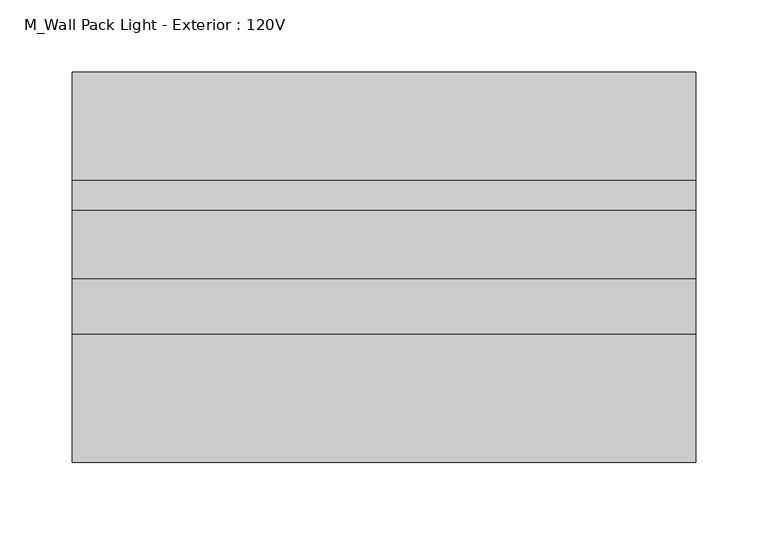
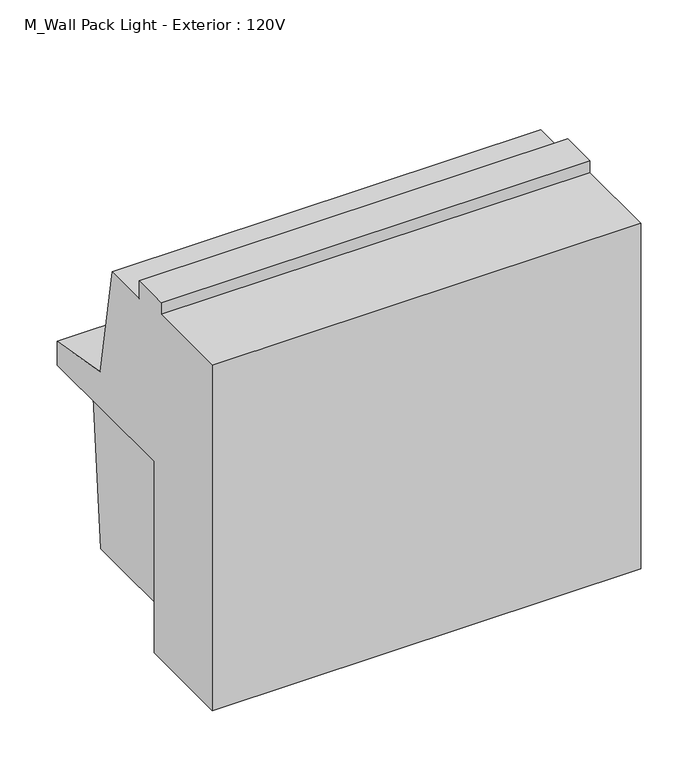
"""IFC4 building model written with IfcOpenShell, lengths in millimetres: light fixture geometry, M_Wall Pack Light - Exterior : 120V."""

import ifcopenshell
import ifcopenshell.guid

model = None  # the IFC model being written
_history = None  # IfcOwnerHistory: only IFC2X3 demands one
_inside = {}  # id of a spatial element -> (the spatial element, [elements in it])
_under = {}  # id of a project, library or spatial element -> (it, [spatial elements below it])
_declared = {}  # id of a project -> (the project, [libraries it declares])
_typed = {}  # id of a type object -> (the type object, [elements of that type])
_made_of = {}  # id of a material, layer set ... -> (it, [elements and type objects made of it])


def new_model(schema):
    """Start an empty IFC model of exactly this schema.

    Asked for "IFC4X3", IfcOpenShell would pick the latest addendum, in which some entities
    have other attributes; the version numbers below select the first issue.
    IFC2X3 requires an IfcOwnerHistory on every rooted entity: one is made here for all.
    """
    global model, _history
    if schema == "IFC4X3":
        model = ifcopenshell.file(schema_version=(4, 3, 0, 0))
    else:
        model = ifcopenshell.file(schema=schema)
    _inside.clear()
    _under.clear()
    _declared.clear()
    _typed.clear()
    _made_of.clear()
    _history = None
    if model.schema == "IFC2X3":
        org = make("IfcOrganization", Name="unknown")
        user = make(
            "IfcPersonAndOrganization",
            ThePerson=make("IfcPerson", FamilyName="unknown"),
            TheOrganization=org,
        )
        app = make(
            "IfcApplication",
            ApplicationDeveloper=org,
            Version="unknown",
            ApplicationFullName="unknown",
            ApplicationIdentifier="unknown",
        )
        _history = make(
            "IfcOwnerHistory",
            OwningUser=user,
            OwningApplication=app,
            ChangeAction="ADDED",
            CreationDate=0,
        )
    return model


def make(cls, **values):
    """One entity of the class cls with the attributes given. An attribute that is None is left unset."""
    return model.create_entity(
        cls, **{name: value for name, value in values.items() if value is not None}
    )


def rooted(cls, **values):
    """An entity with a GlobalId (a new one), such as an element, a storey or a relation."""
    return make(cls, GlobalId=ifcopenshell.guid.new(), OwnerHistory=_history, **values)


def si_unit(unit_type, name, prefix=None):
    """IfcSIUnit, for example si_unit("LENGTHUNIT", "METRE", prefix="MILLI")."""
    return make("IfcSIUnit", UnitType=unit_type, Prefix=prefix, Name=name)


def assignment(units):
    """IfcUnitAssignment: the units of a project."""
    return None if units is None else make("IfcUnitAssignment", Units=units)


def point(xyz):
    """IfcCartesianPoint."""
    return None if xyz is None else make("IfcCartesianPoint", Coordinates=xyz)


def direction(xyz):
    """IfcDirection."""
    return None if xyz is None else make("IfcDirection", DirectionRatios=xyz)


def frame(location, z_axis=None, x_axis=None):
    """IfcAxis2Placement3D, a coordinate frame: its origin and axes. An axis left out is left unset."""
    return make(
        "IfcAxis2Placement3D",
        Location=point(location),
        Axis=direction(z_axis),
        RefDirection=direction(x_axis),
    )


def origin():
    """The frame at (0, 0, 0) with its axes left unset."""
    return frame((0.0, 0.0, 0.0))


def place(relative_to, where):
    """IfcLocalPlacement: puts the frame where relative to a parent placement (None: the world)."""
    return make(
        "IfcLocalPlacement", PlacementRelTo=relative_to, RelativePlacement=where
    )


def context(
    kind, dimensions, precision=None, world=None, true_north=None, identifier=None
):
    """IfcGeometricRepresentationContext, for example the 3D "Model" context."""
    return make(
        "IfcGeometricRepresentationContext",
        ContextIdentifier=identifier,
        ContextType=kind,
        CoordinateSpaceDimension=dimensions,
        Precision=precision,
        WorldCoordinateSystem=world,
        TrueNorth=true_north,
    )


def project(units=None, contexts=None):
    """IfcProject with its units and contexts."""
    return rooted(
        "IfcProject",
        Name="project",
        RepresentationContexts=contexts,
        UnitsInContext=assignment(units),
    )


def spatial(cls, under=None, at=None, **own):
    """A site, building, storey or space (cls), placed at a placement, below another one or the project."""
    s = rooted(cls, ObjectPlacement=at, **own)
    if under is not None:
        _under.setdefault(under.id(), (under, []))[1].append(s)
    return s


def polyline(points):
    """IfcPolyline through the points."""
    return make("IfcPolyline", Points=[point(p) for p in points])


def outline(outer, holes=None, kind="AREA"):
    """IfcArbitraryClosedProfileDef: a profile drawn as a closed curve; with holes, ...WithVoids."""
    if holes is None:
        return make("IfcArbitraryClosedProfileDef", ProfileType=kind, OuterCurve=outer)
    return make(
        "IfcArbitraryProfileDefWithVoids",
        ProfileType=kind,
        OuterCurve=outer,
        InnerCurves=holes,
    )


def extrude(swept, where, along, depth):
    """IfcExtrudedAreaSolid: the profile swept, set in the frame where, extruded along a direction by depth."""
    return make(
        "IfcExtrudedAreaSolid",
        SweptArea=swept,
        Position=where,
        ExtrudedDirection=direction(along),
        Depth=depth,
    )


def shape(context_of_items, identifier, shape_type, items):
    """IfcShapeRepresentation: the items that make up one representation, for example the "Body"."""
    return make(
        "IfcShapeRepresentation",
        ContextOfItems=context_of_items,
        RepresentationIdentifier=identifier,
        RepresentationType=shape_type,
        Items=items,
    )


def source(mapping_origin, context_of_items, identifier, shape_type, items):
    """IfcRepresentationMap: a shape defined once, which mapped items show again and again."""
    return make(
        "IfcRepresentationMap",
        MappingOrigin=mapping_origin,
        MappedRepresentation=shape(context_of_items, identifier, shape_type, items),
    )


def transform(
    local_origin,
    x_axis=None,
    y_axis=None,
    z_axis=None,
    scale=None,
    scale2=None,
    scale3=None,
    uniform=True,
):
    """IfcCartesianTransformationOperator3D, or its non-uniform kind. x_axis, y_axis, z_axis: its Axis1, 2, 3."""
    if uniform:
        return make(
            "IfcCartesianTransformationOperator3D",
            Axis1=direction(x_axis),
            Axis2=direction(y_axis),
            LocalOrigin=point(local_origin),
            Scale=scale,
            Axis3=direction(z_axis),
        )
    return make(
        "IfcCartesianTransformationOperator3DnonUniform",
        Axis1=direction(x_axis),
        Axis2=direction(y_axis),
        LocalOrigin=point(local_origin),
        Scale=scale,
        Axis3=direction(z_axis),
        Scale2=scale2,
        Scale3=scale3,
    )


def mapped(mapping_source, mapping_target):
    """IfcMappedItem: shows the shape of a source again, moved by a transform."""
    return make(
        "IfcMappedItem", MappingSource=mapping_source, MappingTarget=mapping_target
    )


def made_of(thing, what):
    """Note that an element or type object is made of a material, layer set ...; save() writes the relation."""
    if what is not None:
        _made_of.setdefault(what.id(), (what, []))[1].append(thing)
    return thing


def element(
    cls,
    number,
    at=None,
    inside=None,
    cuts=None,
    type_object=None,
    material=None,
    context=None,
    identifier="Body",
    shape_type=None,
    held_by="IfcProductDefinitionShape",
    body=None,
    shapes=None,
    **own,
):
    """One element of the class cls, such as IfcWall. Its Tag is "e" and its number.

    at: its placement. inside: the storey or other place that contains it. cuts: it is an
    opening in that element (IfcRelVoidsElement). A single representation is given by context,
    identifier, shape_type and body (its items); several are given by shapes. held_by: the class
    of the entity that holds the representations. save() writes the other relations.
    """
    e = rooted(cls, Tag="e%d" % number, ObjectPlacement=at, **own)
    if body is not None:
        shapes = [shape(context, identifier, shape_type, body)]
    if shapes is not None:
        e.Representation = make(held_by, Representations=shapes)
    if inside is not None:
        _inside.setdefault(inside.id(), (inside, []))[1].append(e)
    if cuts is not None:
        rooted(
            "IfcRelVoidsElement", RelatingBuildingElement=cuts, RelatedOpeningElement=e
        )
    if type_object is not None:
        _typed.setdefault(type_object.id(), (type_object, []))[1].append(e)
    return made_of(e, material)


def aggregate(whole, parts):
    """IfcRelAggregates: a whole, such as a stair, and the parts it consists of."""
    return rooted("IfcRelAggregates", RelatingObject=whole, RelatedObjects=parts)


def save(model, path):
    """Write the relations noted so far, then the file.

    IfcRelAggregates (storeys below a building ...), IfcRelContainedInSpatialStructure (elements
    in a storey), IfcRelDefinesByType, IfcRelAssociatesMaterial and IfcRelDeclares: one each for
    every whole, place, type object, material and project.
    """
    for whole, parts in _under.values():
        aggregate(whole, parts)
    for where, things in _inside.values():
        rooted(
            "IfcRelContainedInSpatialStructure",
            RelatedElements=things,
            RelatingStructure=where,
        )
    for kind, things in _typed.values():
        rooted("IfcRelDefinesByType", RelatedObjects=things, RelatingType=kind)
    for what, things in _made_of.values():
        rooted("IfcRelAssociatesMaterial", RelatedObjects=things, RelatingMaterial=what)
    for by, libraries in _declared.values():
        rooted("IfcRelDeclares", RelatingContext=by, RelatedDefinitions=libraries)
    model.write(path)


def m_wall_pack_light_exterior_120v_7c12f8c9(model_context):
    return source(origin(), model_context, "Body", "SweptSolid", [
        extrude(outline(polyline([(365.820745, 2350.75), (228.6, 2350.75), (228.6, 2534.9), (380.9170754, 2534.9), (365.820745, 2350.75)])), frame((-68.7349223, 0.0, 0.0), z_axis=(1.0, 0.0, 0.0), x_axis=(0.0, 1.0, 0.0)), (0.0, 0.0, 1.0), 380.9989788),
        extrude(outline(polyline([(215.9, 2712.7), (254.0, 2712.7), (254.0, 2693.65), (301.440971, 2693.65), (322.4426549, 2574.5435323), (397.4850056, 2561.3115412), (397.4850056, 2535.9115412), (228.6, 2535.9115412), (228.6, 2331.7), (127.0, 2331.7), (127.0, 2700.0), (215.9, 2700.0), (215.9, 2712.7)])), frame((-94.1359435, 0.0, 0.0), z_axis=(1.0, 0.0, 0.0), x_axis=(0.0, 1.0, 0.0)), (0.0, 0.0, 1.0), 431.8),
    ])


if __name__ == "__main__":
    model = new_model("IFC4")
    model_context = context("Model", 3, world=origin())
    ifc_project = project(units=[si_unit("LENGTHUNIT", "METRE", prefix="MILLI")], contexts=[model_context])
    site = spatial("IfcSite", under=ifc_project)
    building = spatial("IfcBuilding", under=site)
    placement = place(None, origin())
    m_wall_pack_light_exterior_120v_shape = m_wall_pack_light_exterior_120v_7c12f8c9(model_context)
    element("IfcLightFixture", 1, ObjectType="M_Wall Pack Light - Exterior : 120V", at=placement, inside=building, context=model_context, shape_type="MappedRepresentation", body=[
        mapped(m_wall_pack_light_exterior_120v_shape, transform((0.0, 0.0, 0.0), x_axis=(1.0, 0.0, 0.0), y_axis=(0.0, 1.0, 0.0), z_axis=(0.0, 0.0, 1.0))),
    ])
    save(model, "model.ifc")

# Revit data of these elements
# Type "M_Wall Pack Light - Exterior : 120V"
#   Assembly Code = "D5020230"
#   Wattage = 70 W
#   built-in parameter 1150110 = 1 (stored number, unit not read)
#   built-in parameter 1114217 = 1 (stored number, unit not read)
#   built-in parameter 1150109 = 1 (stored number, unit not read)
#   built-in parameter 1150113 = 1 (stored number, unit not read)
#   built-in parameter 1150115 = 1 (stored number, unit not read)
#   built-in parameter 1150105 = 437.668 (stored number, unit not read)
#   Light Source Symbol Size = 609.6 mm
#   built-in parameter 1150112 = 1 (stored number, unit not read)
#   built-in parameter 1150114 = 1 (stored number, unit not read)
#   built-in parameter 1150107 = 4000 (stored number, unit not read)
#   built-in parameter 1150106 = 4.37668 (stored number, unit not read)
#   built-in parameter 1150104 = 7.29939 (stored number, unit not read)
#   Ballast Voltage = 120 V
#   built-in parameter 1114218 = 1 (stored number, unit not read)
#   built-in parameter 1150133 = 10 (stored number, unit not read)
#   Lumens = 5499.9 lm
#   Mounting Height = 2700 mm
#   Apparent Load = 70 VA
#   built-in parameter 1150134 = 12
#   built-in parameter 1150137 = 1
#   Color Filter = 16777215
#   Ballast Number of Poles = 1
#   Wall Mount Material = Metal - Paint Finish - Dark Grey, Matte
#   Shade Material = Glass
#   Load Classification = Lighting - Exterior
#   Dimming Lamp Color Temperature Shift = (empty or 0)
#   Default Elevation = 0
# Element 1 (IfcLightFixture, "M_Wall Pack Light - Exterior : 120V")
#   Materials on its faces: "Metal - Paint Finish - Dark Grey, Matte", "Glass"
# Materials
#   "Metal - Paint Finish - Dark Grey, Matte": class "Paint", colour RGB 98 98 98, transparency 0
#   "Glass": class "Glass", colour RGB 140 218 255, transparency 0.75, Description = "Soda Lime Glass", Cost = 0
